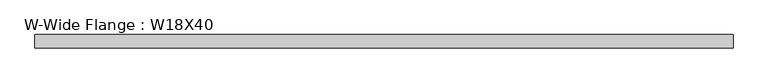
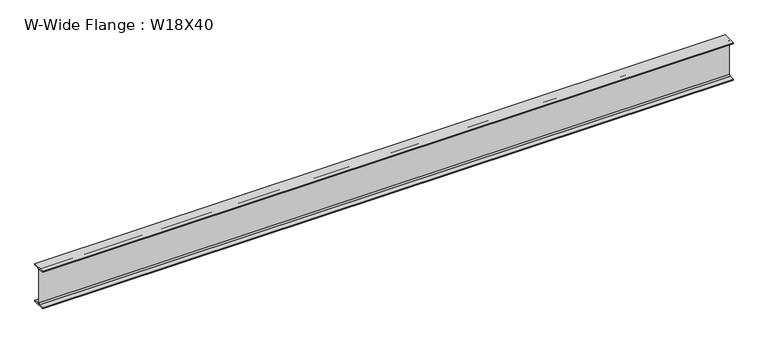
"""IFC4 building model written with IfcOpenShell, lengths in millimetres: beam geometry, W-Wide Flange : W18X40."""

from ifc_helpers import new_model, si_unit, point, frame, frame_2d, origin, place, context, project, spatial, polyline, circle_curve, trimmed, segment, composite_curve, outline, extrude, source, transform, mapped, element, save


def w_wide_flange_w18x40_d6d98870(model_context):
    return source(origin(), model_context, "Body", "SweptSolid", [
        extrude(outline(composite_curve([segment(polyline([(76.454, -213.995), (76.454, -227.33), (-76.454, -227.33), (-76.454, -213.995), (-20.828, -213.995)]), True, "CONTINUOUS"), segment(trimmed(circle_curve(frame_2d((-20.828, -197.1675)), 16.8275), [point((-20.828, -213.995))], [point((-4.0005, -197.1675))], True, "CARTESIAN"), True, "CONTINUOUS"), segment(polyline([(-4.0005, -197.1675), (-4.0005, 197.1675)]), True, "CONTINUOUS"), segment(trimmed(circle_curve(frame_2d((-20.828, 197.1675)), 16.8275), [point((-4.0005, 197.1675))], [point((-20.828, 213.995))], True, "CARTESIAN"), True, "CONTINUOUS"), segment(polyline([(-20.828, 213.995), (-76.454, 213.995), (-76.454, 227.33), (76.454, 227.33), (76.454, 213.995), (20.828, 213.995)]), True, "CONTINUOUS"), segment(trimmed(circle_curve(frame_2d((20.828, 197.1675)), 16.8275), [point((20.828, 213.995))], [point((4.0005, 197.1675))], True, "CARTESIAN"), True, "CONTINUOUS"), segment(polyline([(4.0005, 197.1675), (4.0005, -197.1675)]), True, "CONTINUOUS"), segment(trimmed(circle_curve(frame_2d((20.828, -197.1675)), 16.8275), [point((4.0005, -197.1675))], [point((20.828, -213.995))], True, "CARTESIAN"), True, "CONTINUOUS"), segment(polyline([(20.828, -213.995), (76.454, -213.995)]), True, "CONTINUOUS")], self_intersect=False)), frame((-3917.95, 0.0, 0.0), z_axis=(1.0, 0.0, 0.0), x_axis=(0.0, 1.0, 0.0)), (0.0, 0.0, 1.0), 7897.8125),
    ])


if __name__ == "__main__":
    model = new_model("IFC4")
    model_context = context("Model", 3, world=origin())
    ifc_project = project(units=[si_unit("LENGTHUNIT", "METRE", prefix="MILLI")], contexts=[model_context])
    site = spatial("IfcSite", under=ifc_project)
    building = spatial("IfcBuilding", under=site)
    placement = place(None, origin())
    w_wide_flange_w18x40_shape = w_wide_flange_w18x40_d6d98870(model_context)
    element("IfcBeam", 1, ObjectType="W-Wide Flange : W18X40", at=placement, inside=building, context=model_context, shape_type="MappedRepresentation", body=[
        mapped(w_wide_flange_w18x40_shape, transform((0.0, 0.0, 0.0), x_axis=(1.0, 0.0, 0.0), y_axis=(0.0, 1.0, 0.0), z_axis=(0.0, 0.0, 1.0))),
    ])
    save(model, "model.ifc")

# Revit data of these elements
# Type "W-Wide Flange : W18X40"
#   Assembly Code = "B10"
#   W = 40
#   Length [instance default] = 5' - 0"
#   bf = 0' - 6.02"
#   d = 1' - 5.9"
#   k = 0' - 1 3/16"
#   k2 = 0' - 0.6625"
#   tf = 0' - 0.525"
#   tw = 0' - 0.315"
#   A = 0.0819444 SF
#   Structural Material [instance default] = Steel ASTM A992
# Element 1 (IfcBeam, "W-Wide Flange : W18X40")
#   Materials on its faces: "Steel ASTM A992"
# Materials
#   "Steel ASTM A992": class "Metal", colour RGB 199 199 199, transparency 0, Description = "Structural steel 50ksi", Cost = 0
